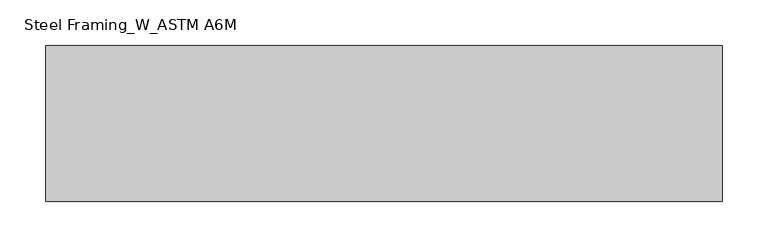
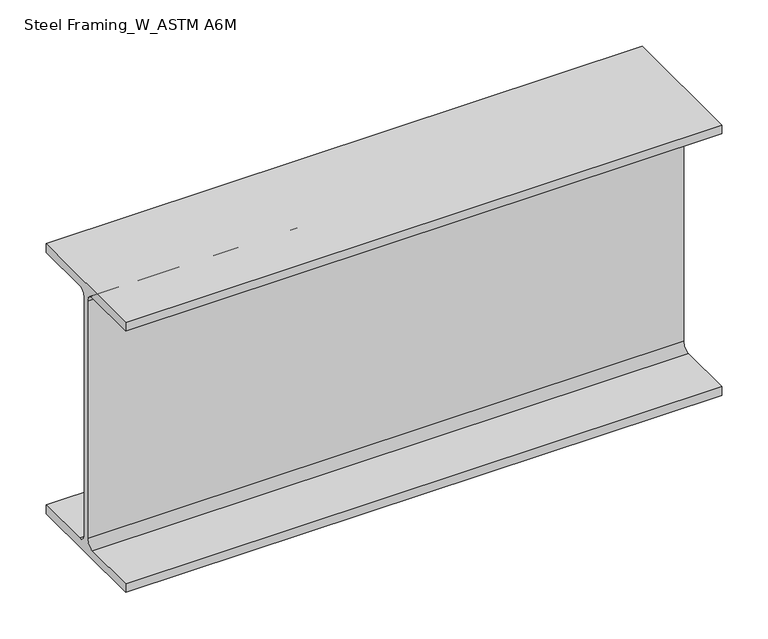
"""IFC4 building model written with IfcOpenShell, lengths in millimetres: beam geometry, Steel Framing_W_ASTM A6M : H_SB_AR_S02_W360x51_RG1."""

from ifc_helpers import new_model, si_unit, point, frame, frame_2d, origin, place, context, project, spatial, polyline, circle_curve, trimmed, segment, composite_curve, outline, extrude, source, transform, mapped, element, save


def steel_framing_w_astm_a6m_a80668d3(model_context):
    return source(origin(), model_context, "Body", "SweptSolid", [
        extrude(outline(composite_curve([segment(polyline([(85.5, -166.4), (85.5, -178.0), (-85.5, -178.0), (-85.5, -166.4), (-13.72, -166.4)]), True, "CONTINUOUS"), segment(trimmed(circle_curve(frame_2d((-13.72, -156.3)), 10.1), [point((-13.72, -166.4))], [point((-3.62, -156.3))], True, "CARTESIAN"), True, "CONTINUOUS"), segment(polyline([(-3.62, -156.3), (-3.62, 156.3)]), True, "CONTINUOUS"), segment(trimmed(circle_curve(frame_2d((-13.72, 156.3)), 10.1), [point((-3.62, 156.3))], [point((-13.72, 166.4))], True, "CARTESIAN"), True, "CONTINUOUS"), segment(polyline([(-13.72, 166.4), (-85.5, 166.4), (-85.5, 178.0), (85.5, 178.0), (85.5, 166.4), (13.72, 166.4)]), True, "CONTINUOUS"), segment(trimmed(circle_curve(frame_2d((13.72, 156.3)), 10.1), [point((13.72, 166.4))], [point((3.62, 156.3))], True, "CARTESIAN"), True, "CONTINUOUS"), segment(polyline([(3.62, 156.3), (3.62, -156.3)]), True, "CONTINUOUS"), segment(trimmed(circle_curve(frame_2d((13.72, -156.3)), 10.1), [point((3.62, -156.3))], [point((13.72, -166.4))], True, "CARTESIAN"), True, "CONTINUOUS"), segment(polyline([(13.72, -166.4), (85.5, -166.4)]), True, "CONTINUOUS")], self_intersect=False)), frame((-493.5, 0.0, 0.0), z_axis=(1.0, 0.0, 0.0), x_axis=(0.0, 1.0, 0.0)), (0.0, 0.0, 1.0), 742.0),
    ])


if __name__ == "__main__":
    model = new_model("IFC4")
    model_context = context("Model", 3, world=origin())
    ifc_project = project(units=[si_unit("LENGTHUNIT", "METRE", prefix="MILLI")], contexts=[model_context])
    site = spatial("IfcSite", under=ifc_project)
    building = spatial("IfcBuilding", under=site)
    placement = place(None, origin())
    steel_framing_w_astm_a6m_shape = steel_framing_w_astm_a6m_a80668d3(model_context)
    element("IfcBeam", 1, ObjectType="Steel Framing_W_ASTM A6M : H_SB_AR_S02_W360x51_RG1", at=placement, inside=building, context=model_context, shape_type="MappedRepresentation", body=[
        mapped(steel_framing_w_astm_a6m_shape, transform((0.0, 0.0, 0.0), x_axis=(1.0, 0.0, 0.0), y_axis=(0.0, 1.0, 0.0), z_axis=(0.0, 0.0, 1.0))),
    ])
    save(model, "model.ifc")

# Revit data of these elements
# Type "Steel Framing_W_ASTM A6M : H_SB_AR_S02_W360x51_RG1"
#   Type Mark = "RG1"
#   Section Name Key = "W14x34"
#   Width = 17.1 cm
#   Web Thickness = 0.724 cm
#   Web Fillet = 1.01 cm
#   Warping Constant = 287000.0 cm⁶
#   Torsional Moment of Inertia = 23.70 cm⁴
#   Section Area = 64.5 cm²
#   Plastic Modulus weak axis = 174.0 cm³
#   Plastic Modulus strong axis = 895.0 cm³
#   Perimeter = 1.36 m²/m
#   Nominal Weight = 51.00 kgf/m
#   Moment of Inertia weak axis = 970.00 cm⁴
#   Moment of Inertia strong axis = 14200.00 cm⁴
#   Height = 35.6 cm
#   Flange Thickness = 1.16 cm
#   Elastic Modulus weak axis = 113.0 cm³
#   Elastic Modulus strong axis = 796.0 cm³
#   Centroid Vertical = 17.8 cm
#   Centroid Horizontal = 8.55 cm
#   Length [instance default] = 1500 mm
#   Structural Material [instance default] = Steel, 45-345
#   Bolt Spacing = 0
#   Assembly Code = ""
# Element 1 (IfcBeam, "Steel Framing_W_ASTM A6M : H_SB_AR_S02_W360x51_RG1")
#   Materials on its faces: "Steel, 45-345"
# Materials
#   "Steel, 45-345": class "Metal", colour RGB 189 187 185, transparency 0, Description = "Steel 345 MPa", Cost = 0
